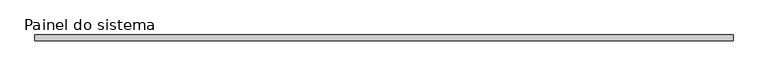
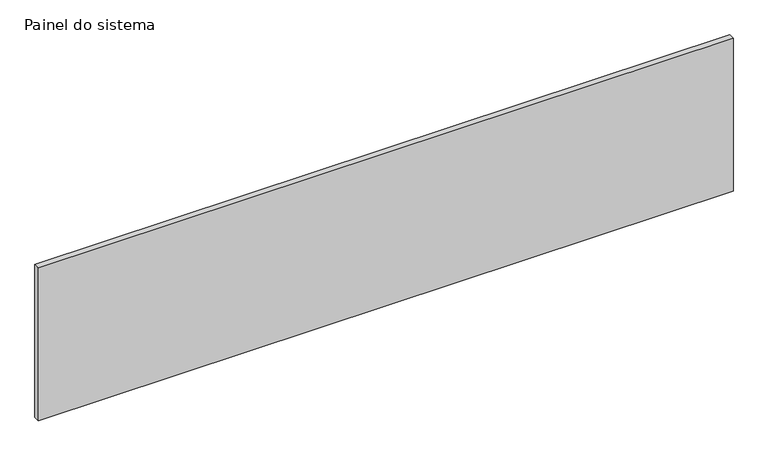
"""IFC4 building model written with IfcOpenShell, lengths in millimetres: plate geometry, Painel do sistema : Envidraçado."""

from ifc_helpers import new_model, si_unit, origin, origin_with_axes, place, context, project, spatial, polyline, outline, extrude, source, transform, mapped, element, save


def painel_do_sistema_14e00207(model_context):
    return source(origin(), model_context, "Body", "SweptSolid", [
        extrude(outline(polyline([(1475.0, 24.5), (-1475.0, 24.5), (-1475.0, 49.5), (1475.0, 49.5), (1475.0, 24.5)])), origin_with_axes(), (0.0, 0.0, 1.0), 685.7133319),
    ])


if __name__ == "__main__":
    model = new_model("IFC4")
    model_context = context("Model", 3, world=origin())
    ifc_project = project(units=[si_unit("LENGTHUNIT", "METRE", prefix="MILLI")], contexts=[model_context])
    site = spatial("IfcSite", under=ifc_project)
    building = spatial("IfcBuilding", under=site)
    placement = place(None, origin())
    painel_do_sistema_shape = painel_do_sistema_14e00207(model_context)
    element("IfcPlate", 1, ObjectType="Painel do sistema : Envidraçado", at=placement, inside=building, context=model_context, shape_type="MappedRepresentation", body=[
        mapped(painel_do_sistema_shape, transform((0.0, 0.0, 0.0), x_axis=(1.0, 0.0, 0.0), y_axis=(0.0, 1.0, 0.0), z_axis=(0.0, 0.0, 1.0))),
    ])
    save(model, "model.ifc")

# Revit data of these elements
# Type "Painel do sistema : Envidraçado"
#   Construction Type Id = "GSP4R"
#   Analytic Construction = "Vidraça única Pilkington 1/8 pol"
#   Visual Light Transmittance = 0.9
#   Solar Heat Gain Coefficient = 0.86
#   Heat Transfer Coefficient (U) = 6.7069 W/(m²·K)
# Element 1 (IfcPlate, "Painel do sistema : Envidraçado")
#   Materials on its faces: "Vidro"
# Materials
#   "Vidro": class "Vidro", colour RGB 0 128 192, transparency 0.9, Description = "Vidro de sílica", Cost = 0
